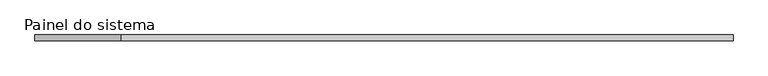
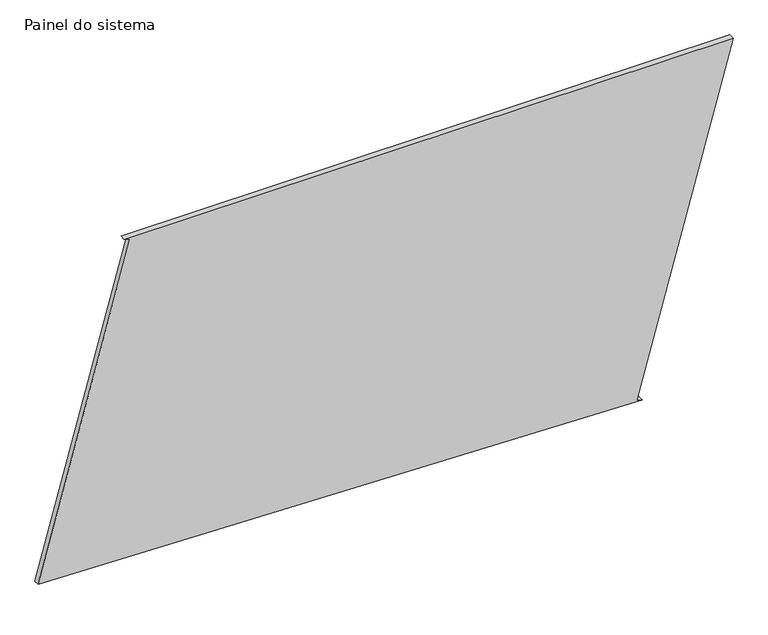
"""IFC4 building model written with IfcOpenShell, lengths in millimetres: plate geometry, Painel do sistema : Envidraçado."""

from ifc_helpers import new_model, si_unit, frame, origin, place, context, project, spatial, polyline, outline, extrude, source, transform, mapped, element, save


def painel_do_sistema_40c64ab4(model_context):
    return source(origin(), model_context, "Body", "SweptSolid", [
        extrude(outline(polyline([(0.0, 1114.7117205), (6.6310485, 1090.6071733), (1524.0167031, 1508.0328924), (1524.0167031, -1134.2371721), (1517.3856545, -1110.1326249), (70.9770358, -1508.0328924), (0.0, 1114.7117205)])), frame((0.0, 24.5, 0.0), z_axis=(0.0, 1.0, 0.0), x_axis=(0.0, 0.0, 1.0)), (0.0, 0.0, 1.0), 25.0),
    ])


if __name__ == "__main__":
    model = new_model("IFC4")
    model_context = context("Model", 3, world=origin())
    ifc_project = project(units=[si_unit("LENGTHUNIT", "METRE", prefix="MILLI")], contexts=[model_context])
    site = spatial("IfcSite", under=ifc_project)
    building = spatial("IfcBuilding", under=site)
    placement = place(None, origin())
    painel_do_sistema_shape = painel_do_sistema_40c64ab4(model_context)
    element("IfcPlate", 1, ObjectType="Painel do sistema : Envidraçado", at=placement, inside=building, context=model_context, shape_type="MappedRepresentation", body=[
        mapped(painel_do_sistema_shape, transform((0.0, 0.0, 0.0), x_axis=(1.0, 0.0, 0.0), y_axis=(0.0, 1.0, 0.0), z_axis=(0.0, 0.0, 1.0))),
    ])
    save(model, "model.ifc")

# Revit data of these elements
# Type "Painel do sistema : Envidraçado"
#   Construction Type Id = "GSP4R"
#   Analytic Construction = "Vidraça única Pilkington 1/8 pol"
#   Visual Light Transmittance = 0.9
#   Solar Heat Gain Coefficient = 0.86
#   Heat Transfer Coefficient (U) = 6.7069 W/(m²·K)
# Element 1 (IfcPlate, "Painel do sistema : Envidraçado")
#   Materials on its faces: "Vidro"
# Materials
#   "Vidro": class "Vidro", colour RGB 0 128 192, transparency 0.9, Description = "Vidro de sílica", Cost = 0
